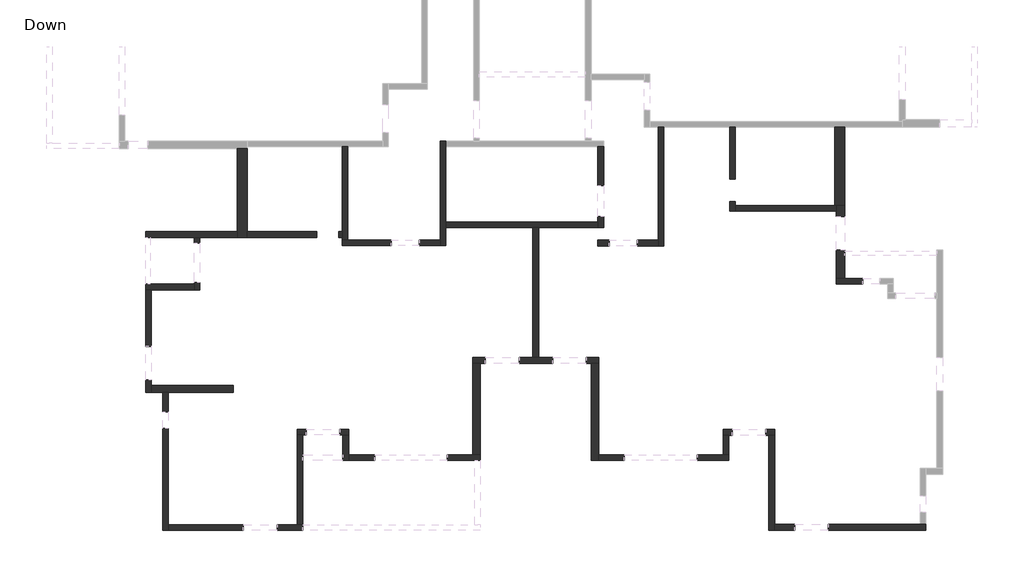
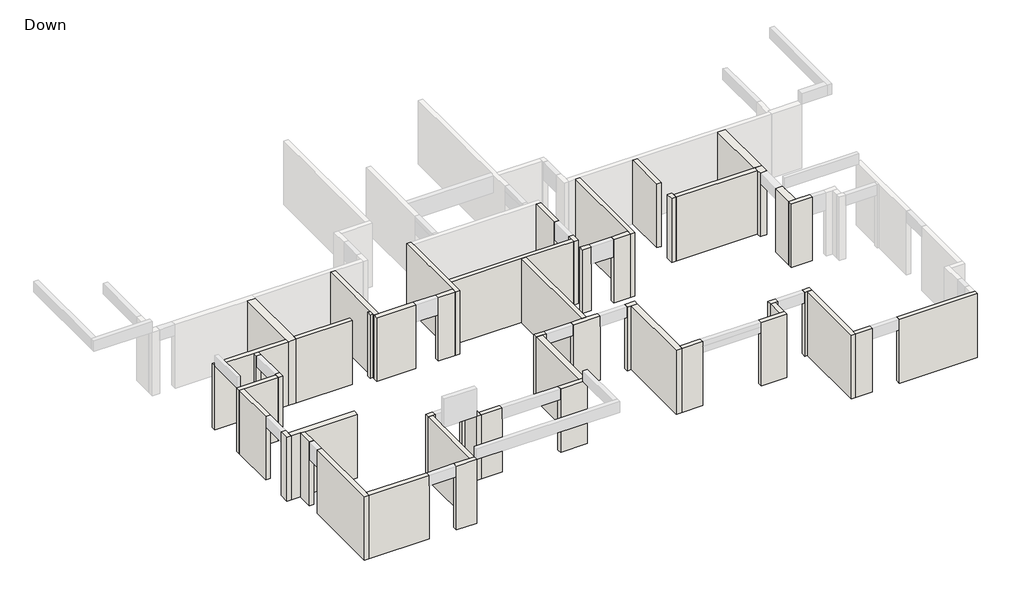
# One storey, part 1 of 3: 51 walls.
# Revit data of these elements (continued)
# Element 32 (IfcWall, "20") (continued)
#   Base Offset = 0 cm
#   wall height = 300 cm
#   SOFiSTiK_AMG_Scheduled = yes
#   SOFiSTiK_AMG_Adjusted = yes
#   Phase Created = New Construction
#   Base Constraint = Down
#   Top Constraint = Typical Floor
#   Materials on its faces: "Concrete"
# Element 33 (IfcWall, "20")
#   Comments = ""
#   Mark = "W67"
#   SOFiSTiK_EdgeZones = "W67"
#   SOFiSTiK_AMG_Comments = ""
#   Top Offset = 0 cm
#   Base Offset = 0 cm
#   wall height = 300 cm
#   SOFiSTiK_AMG_Scheduled = yes
#   SOFiSTiK_AMG_Adjusted = yes
#   Phase Created = New Construction
#   Base Constraint = Down
#   Top Constraint = Typical Floor
#   Materials on its faces: "Concrete"
# Element 34 (IfcWall, "20")
#   Comments = ""
#   Mark = "W68"
#   SOFiSTiK_EdgeZones = "W68"
#   SOFiSTiK_AMG_Comments = ""
#   Top Offset = 0 cm
#   Base Offset = 0 cm
#   wall height = 300 cm
#   SOFiSTiK_AMG_Scheduled = yes
#   SOFiSTiK_AMG_Adjusted = yes
#   Phase Created = New Construction
#   Base Constraint = Down
#   Top Constraint = Typical Floor
#   Materials on its faces: "Concrete"
# Element 35 (IfcWall, "20")
#   Comments = ""
#   Mark = "W69"
#   SOFiSTiK_EdgeZones = "W69"
#   SOFiSTiK_AMG_Comments = ""
#   Top Offset = 0 cm
#   Base Offset = 0 cm
#   wall height = 300 cm
#   SOFiSTiK_AMG_Scheduled = yes
#   SOFiSTiK_AMG_Adjusted = yes
#   Phase Created = New Construction
#   Base Constraint = Down
#   Top Constraint = Typical Floor
#   Materials on its faces: "Concrete"
# Element 36 (IfcWall, "20")
#   Comments = ""
#   Mark = "W70"
#   SOFiSTiK_EdgeZones = "W70"
#   SOFiSTiK_AMG_Comments = ""
#   Top Offset = 0 cm
#   Base Offset = 0 cm
#   wall height = 300 cm
#   SOFiSTiK_AMG_Scheduled = yes
#   SOFiSTiK_AMG_Adjusted = yes
#   Phase Created = New Construction
#   Base Constraint = Down
#   Top Constraint = Typical Floor
#   Materials on its faces: "Concrete"
# Element 37 (IfcWall, "20")
#   Comments = ""
#   Mark = "W80"
#   SOFiSTiK_EdgeZones = "W80"
#   SOFiSTiK_AMG_Comments = ""
#   Top Offset = 0 cm
#   Base Offset = 0 cm
#   wall height = 300 cm
#   SOFiSTiK_AMG_Scheduled = yes
#   SOFiSTiK_AMG_Adjusted = yes
#   Phase Created = New Construction
#   Base Constraint = Down
#   Top Constraint = Typical Floor
#   Materials on its faces: "Concrete"
# Element 38 (IfcWall, "20")
#   Comments = ""
#   Mark = "W81"
#   SOFiSTiK_EdgeZones = "W81"
#   SOFiSTiK_AMG_Comments = ""
#   Top Offset = 0 cm
#   Base Offset = 0 cm
#   wall height = 300 cm
#   SOFiSTiK_AMG_Scheduled = yes
#   SOFiSTiK_AMG_Adjusted = yes
#   Phase Created = New Construction
#   Base Constraint = Down
#   Top Constraint = Typical Floor
#   Materials on its faces: "Concrete"
# Element 39 (IfcWall, "20")
#   Comments = ""
#   Mark = "W82"
#   SOFiSTiK_EdgeZones = "W82"
#   SOFiSTiK_AMG_Comments = ""
#   Top Offset = 0 cm
#   Base Offset = 0 cm
#   wall height = 300 cm
#   SOFiSTiK_AMG_Scheduled = yes
#   SOFiSTiK_AMG_Adjusted = yes
#   Phase Created = New Construction
#   Base Constraint = Down
#   Top Constraint = Typical Floor
#   Materials on its faces: "Concrete"
# Element 40 (IfcWall, "20")
#   Comments = ""
#   Mark = "W83"
#   SOFiSTiK_EdgeZones = "W83"
#   SOFiSTiK_AMG_Comments = ""
#   Top Offset = 0 cm
#   Base Offset = 0 cm
#   wall height = 300 cm
#   SOFiSTiK_AMG_Scheduled = yes
#   SOFiSTiK_AMG_Adjusted = yes
#   Phase Created = New Construction
#   Base Constraint = Down
#   Top Constraint = Typical Floor
#   Materials on its faces: "Concrete"
# Element 41 (IfcWall, "20")
#   Comments = ""
#   Mark = "W101"
#   SOFiSTiK_EdgeZones = "W101"
#   SOFiSTiK_AMG_Comments = ""
#   Top Offset = 0 cm
#   Base Offset = 0 cm
#   wall height = 300 cm
#   SOFiSTiK_AMG_Scheduled = yes
#   SOFiSTiK_AMG_Adjusted = yes
#   Phase Created = New Construction
#   Base Constraint = Down
#   Top Constraint = Typical Floor
#   Materials on its faces: "Concrete"
# Element 42 (IfcWall, "20")
#   Comments = ""
#   Mark = "W102"
#   SOFiSTiK_EdgeZones = "W102"
#   SOFiSTiK_AMG_Comments = ""
#   Top Offset = 0 cm
#   Base Offset = 0 cm
#   wall height = 300 cm
#   SOFiSTiK_AMG_Scheduled = yes
#   SOFiSTiK_AMG_Adjusted = yes
#   Phase Created = New Construction
#   Base Constraint = Down
#   Top Constraint = Typical Floor
#   Materials on its faces: "Concrete"
# Element 43 (IfcWall, "20")
#   Comments = ""
#   Mark = "W103"
#   SOFiSTiK_EdgeZones = "W103"
#   SOFiSTiK_AMG_Comments = ""
#   Top Offset = 0 cm
#   Base Offset = 0 cm
#   wall height = 300 cm
#   SOFiSTiK_AMG_Scheduled = yes
#   SOFiSTiK_AMG_Adjusted = yes
#   Phase Created = New Construction
#   Base Constraint = Down
#   Top Constraint = Typical Floor
#   Materials on its faces: "Concrete"
# Element 44 (IfcWall, "20")
#   Comments = ""
#   Mark = "W104"
#   SOFiSTiK_EdgeZones = "W104"
#   SOFiSTiK_AMG_Comments = ""
#   Top Offset = 0 cm
#   Base Offset = 0 cm
#   wall height = 300 cm
#   SOFiSTiK_AMG_Scheduled = yes
#   SOFiSTiK_AMG_Adjusted = yes
#   Phase Created = New Construction
#   Base Constraint = Down
#   Top Constraint = Typical Floor
#   Materials on its faces: "Concrete"
# Element 45 (IfcWall, "25")
#   Comments = ""
#   Mark = "W116"
#   SOFiSTiK_EdgeZones = "W116"
#   SOFiSTiK_AMG_Comments = ""
#   Top Offset = 0 cm
#   Base Offset = 0 cm
#   wall height = 300 cm
#   SOFiSTiK_AMG_Scheduled = yes
#   SOFiSTiK_AMG_Adjusted = yes
#   Phase Created = New Construction
#   Base Constraint = Down
#   Top Constraint = Typical Floor
#   Materials on its faces: "Concrete"
# Element 46 (IfcWall, "27")
#   Comments = ""
#   Mark = "W110"
#   SOFiSTiK_EdgeZones = "W110"
#   SOFiSTiK_AMG_Comments = ""
#   Top Offset = 0 cm
#   Base Offset = 0 cm
#   wall height = 300 cm
#   SOFiSTiK_AMG_Scheduled = yes
#   SOFiSTiK_AMG_Adjusted = yes
#   Phase Created = New Construction
#   Base Constraint = Down
#   Top Constraint = Typical Floor
#   Materials on its faces: "Concrete"
# Element 47 (IfcWall, "27")
#   Comments = ""
#   Mark = "W111"
#   SOFiSTiK_EdgeZones = "W111"
#   SOFiSTiK_AMG_Comments = ""
#   Top Offset = 0 cm
#   Base Offset = 0 cm
#   wall height = 300 cm
#   SOFiSTiK_AMG_Scheduled = yes
#   SOFiSTiK_AMG_Adjusted = yes
#   Phase Created = New Construction
#   Base Constraint = Down
#   Top Constraint = Typical Floor
#   Materials on its faces: "Concrete"
# Element 48 (IfcWall, "30")
#   Comments = ""
#   Mark = "W120"
#   SOFiSTiK_EdgeZones = "W120"
#   SOFiSTiK_AMG_Comments = ""
#   Top Offset = 0 cm
#   Base Offset = 0 cm
#   wall height = 300 cm
#   SOFiSTiK_AMG_Scheduled = yes
#   SOFiSTiK_AMG_Adjusted = yes
#   Phase Created = New Construction
#   Base Constraint = Down
#   Top Constraint = Typical Floor
#   Materials on its faces: "Concrete"
# Element 49 (IfcWall, "30")
#   Comments = ""
#   Mark = "W121"
#   SOFiSTiK_EdgeZones = "W121"
#   SOFiSTiK_AMG_Comments = ""
#   Top Offset = 0 cm
#   Base Offset = 0 cm
#   wall height = 300 cm
#   SOFiSTiK_AMG_Scheduled = yes
#   SOFiSTiK_AMG_Adjusted = yes
#   Phase Created = New Construction
#   Base Constraint = Down
#   Top Constraint = Typical Floor
#   Materials on its faces: "Concrete"
# Element 50 (IfcWall, "35")
#   Comments = ""
#   Mark = "W2"
#   SOFiSTiK_EdgeZones = "W2"
#   SOFiSTiK_AMG_Comments = ""
#   Top Offset = 0 cm
#   Base Offset = 0 cm
#   wall height = 300 cm
#   SOFiSTiK_AMG_Scheduled = yes
#   SOFiSTiK_AMG_Adjusted = yes
#   Phase Created = New Construction
#   Base Constraint = Down
#   Top Constraint = Typical Floor
#   Materials on its faces: "Concrete"
# Element 51 (IfcWall, "35")
#   Comments = ""
#   Mark = "W4"
#   SOFiSTiK_EdgeZones = "W4"
#   SOFiSTiK_AMG_Comments = ""
#   Top Offset = 0 cm
#   Base Offset = 0 cm
#   wall height = 300 cm
#   SOFiSTiK_AMG_Scheduled = yes
#   SOFiSTiK_AMG_Adjusted = yes
#   Phase Created = New Construction
#   Base Constraint = Down
#   Top Constraint = Typical Floor
#   Materials on its faces: "Concrete"
# Materials
#   "Concrete": class "Concrete", colour RGB 192 192 192, transparency 0, Keynote = "01000", Description = "Cast-in-place concrete", Cost = 0
